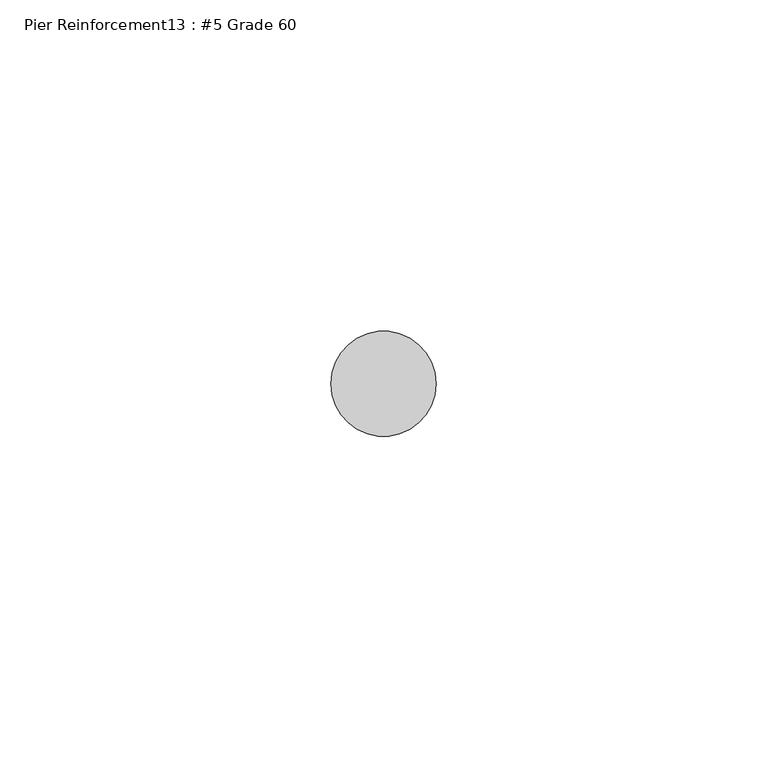
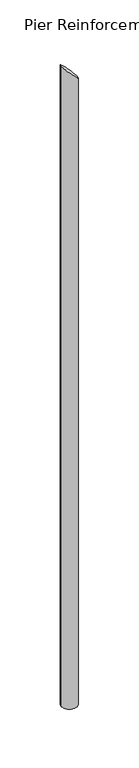
"""IFC4 building model written with IfcOpenShell, lengths in millimetres: proxy geometry, Pier Reinforcement13 : #5 Grade 60."""

from ifc_helpers import new_model, si_unit, frame, origin, place, context, project, spatial, circle_curve, ellipse_curve, source, transform, mapped, element, save
from ifc_brep_helpers import plane_surface, cylinder_surface, advanced_brep


def pier_reinforcement13_5_grade_60_ff8834b7(model_context):
    return source(origin(), model_context, "Body", "AdvancedBrep", [
        advanced_brep(
        [(587484.5778122, -534096.6663841, -733.425), (587500.4528122, -534096.6663841, -733.425), (587500.4528122, -534096.6663841, -63.5), (587484.5778122, -534096.6663841, -47.625)],
        [
            (0, 1, circle_curve(frame((587492.5153122, -534096.6663841, -733.425), z_axis=(0.0, 0.0, -1.0), x_axis=(-1.0, 0.0, 0.0)), 7.9375)),
            (1, 0, circle_curve(frame((587492.5153122, -534096.6663841, -733.425), z_axis=(0.0, 0.0, -1.0), x_axis=(-1.0, 0.0, 0.0)), 7.9375)),
            (1, 2),
            (2, 3, ellipse_curve(frame((587492.5153122, -534096.6663841, -55.5625), z_axis=(-0.7071067811865458, 0.0, -0.7071067811865493), x_axis=(-0.7071067811865493, 0.0, 0.7071067811865456)), 11.2253202, 7.9375)),
            (3, 0),
            (3, 2, ellipse_curve(frame((587492.5153122, -534096.6663841, -55.5625), z_axis=(-0.7071067811865458, 0.0, -0.7071067811865493), x_axis=(-0.7071067811865493, 0.0, 0.7071067811865456)), 11.2253202, 7.9375)),
        ],
        [
            plane_surface(frame((587484.5778122, -534096.6663841, -733.425), z_axis=(0.0, 0.0, -1.0), x_axis=(0.0, 1.0, 0.0))),
            cylinder_surface(frame((587492.5153122, -534096.6663841, -733.425), z_axis=(0.0, 0.0, 1.0), x_axis=(-1.0, 0.0, 0.0)), 7.9375),
            plane_surface(frame((587484.5778122, -534071.2663841, -47.625), z_axis=(0.7071067811865458, 0.0, 0.7071067811865493), x_axis=(0.0, -1.0, 0.0))),
        ],
        [
            (0, [[1, 2]]),
            (1, [[-2, 3, 4, 5]]),
            (1, [[-1, -5, 6, -3]]),
            (2, [[-4, -6]]),
        ],
    ),
    ])


if __name__ == "__main__":
    model = new_model("IFC4")
    model_context = context("Model", 3, world=origin())
    ifc_project = project(units=[si_unit("LENGTHUNIT", "METRE", prefix="MILLI")], contexts=[model_context])
    site = spatial("IfcSite", under=ifc_project)
    building = spatial("IfcBuilding", under=site)
    placement = place(None, origin())
    pier_reinforcement13_5_grade_60_shape = pier_reinforcement13_5_grade_60_ff8834b7(model_context)
    element("IfcBuildingElementProxy", 1, Name="Pier Reinforcement13 : #5 Grade 60", ObjectType="Pier Reinforcement13 : #5 Grade 60", at=placement, inside=building, context=model_context, shape_type="MappedRepresentation", body=[
        mapped(pier_reinforcement13_5_grade_60_shape, transform((0.0, 0.0, 0.0), x_axis=(1.0, 0.0, 0.0), y_axis=(0.0, 1.0, 0.0), z_axis=(0.0, 0.0, 1.0))),
    ])
    save(model, "model.ifc")

# Revit data of these elements
# Element 1 (IfcBuildingElementProxy, "Pier Reinforcement13 : #5 Grade 60")
#   Materials on its faces: "#4 GR. 60 REINF. @ 16\" O.C. EW."
# Materials
#   "#4 GR. 60 REINF. @ 16\" O.C. EW.": class "Generic", colour RGB 84 83 81, transparency 0, Cost = 0
